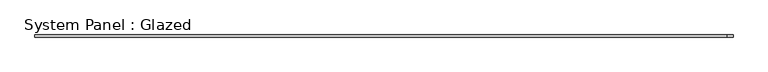
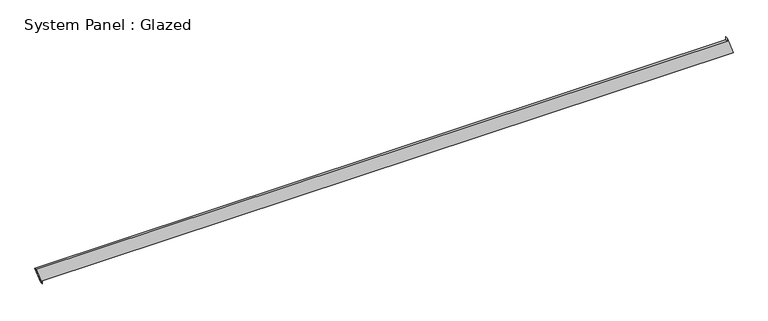
"""IFC4 building model written with IfcOpenShell, lengths in millimetres: plate geometry, System Panel : Glazed."""

import ifcopenshell
import ifcopenshell.guid

model = None  # the IFC model being written
_history = None  # IfcOwnerHistory: only IFC2X3 demands one
_inside = {}  # id of a spatial element -> (the spatial element, [elements in it])
_under = {}  # id of a project, library or spatial element -> (it, [spatial elements below it])
_declared = {}  # id of a project -> (the project, [libraries it declares])
_typed = {}  # id of a type object -> (the type object, [elements of that type])
_made_of = {}  # id of a material, layer set ... -> (it, [elements and type objects made of it])


def new_model(schema):
    """Start an empty IFC model of exactly this schema.

    Asked for "IFC4X3", IfcOpenShell would pick the latest addendum, in which some entities
    have other attributes; the version numbers below select the first issue.
    IFC2X3 requires an IfcOwnerHistory on every rooted entity: one is made here for all.
    """
    global model, _history
    if schema == "IFC4X3":
        model = ifcopenshell.file(schema_version=(4, 3, 0, 0))
    else:
        model = ifcopenshell.file(schema=schema)
    _inside.clear()
    _under.clear()
    _declared.clear()
    _typed.clear()
    _made_of.clear()
    _history = None
    if model.schema == "IFC2X3":
        org = make("IfcOrganization", Name="unknown")
        user = make(
            "IfcPersonAndOrganization",
            ThePerson=make("IfcPerson", FamilyName="unknown"),
            TheOrganization=org,
        )
        app = make(
            "IfcApplication",
            ApplicationDeveloper=org,
            Version="unknown",
            ApplicationFullName="unknown",
            ApplicationIdentifier="unknown",
        )
        _history = make(
            "IfcOwnerHistory",
            OwningUser=user,
            OwningApplication=app,
            ChangeAction="ADDED",
            CreationDate=0,
        )
    return model


def make(cls, **values):
    """One entity of the class cls with the attributes given. An attribute that is None is left unset."""
    return model.create_entity(
        cls, **{name: value for name, value in values.items() if value is not None}
    )


def rooted(cls, **values):
    """An entity with a GlobalId (a new one), such as an element, a storey or a relation."""
    return make(cls, GlobalId=ifcopenshell.guid.new(), OwnerHistory=_history, **values)


def si_unit(unit_type, name, prefix=None):
    """IfcSIUnit, for example si_unit("LENGTHUNIT", "METRE", prefix="MILLI")."""
    return make("IfcSIUnit", UnitType=unit_type, Prefix=prefix, Name=name)


def assignment(units):
    """IfcUnitAssignment: the units of a project."""
    return None if units is None else make("IfcUnitAssignment", Units=units)


def point(xyz):
    """IfcCartesianPoint."""
    return None if xyz is None else make("IfcCartesianPoint", Coordinates=xyz)


def direction(xyz):
    """IfcDirection."""
    return None if xyz is None else make("IfcDirection", DirectionRatios=xyz)


def frame(location, z_axis=None, x_axis=None):
    """IfcAxis2Placement3D, a coordinate frame: its origin and axes. An axis left out is left unset."""
    return make(
        "IfcAxis2Placement3D",
        Location=point(location),
        Axis=direction(z_axis),
        RefDirection=direction(x_axis),
    )


def origin():
    """The frame at (0, 0, 0) with its axes left unset."""
    return frame((0.0, 0.0, 0.0))


def place(relative_to, where):
    """IfcLocalPlacement: puts the frame where relative to a parent placement (None: the world)."""
    return make(
        "IfcLocalPlacement", PlacementRelTo=relative_to, RelativePlacement=where
    )


def context(
    kind, dimensions, precision=None, world=None, true_north=None, identifier=None
):
    """IfcGeometricRepresentationContext, for example the 3D "Model" context."""
    return make(
        "IfcGeometricRepresentationContext",
        ContextIdentifier=identifier,
        ContextType=kind,
        CoordinateSpaceDimension=dimensions,
        Precision=precision,
        WorldCoordinateSystem=world,
        TrueNorth=true_north,
    )


def project(units=None, contexts=None):
    """IfcProject with its units and contexts."""
    return rooted(
        "IfcProject",
        Name="project",
        RepresentationContexts=contexts,
        UnitsInContext=assignment(units),
    )


def spatial(cls, under=None, at=None, **own):
    """A site, building, storey or space (cls), placed at a placement, below another one or the project."""
    s = rooted(cls, ObjectPlacement=at, **own)
    if under is not None:
        _under.setdefault(under.id(), (under, []))[1].append(s)
    return s


def polyline(points):
    """IfcPolyline through the points."""
    return make("IfcPolyline", Points=[point(p) for p in points])


def outline(outer, holes=None, kind="AREA"):
    """IfcArbitraryClosedProfileDef: a profile drawn as a closed curve; with holes, ...WithVoids."""
    if holes is None:
        return make("IfcArbitraryClosedProfileDef", ProfileType=kind, OuterCurve=outer)
    return make(
        "IfcArbitraryProfileDefWithVoids",
        ProfileType=kind,
        OuterCurve=outer,
        InnerCurves=holes,
    )


def extrude(swept, where, along, depth):
    """IfcExtrudedAreaSolid: the profile swept, set in the frame where, extruded along a direction by depth."""
    return make(
        "IfcExtrudedAreaSolid",
        SweptArea=swept,
        Position=where,
        ExtrudedDirection=direction(along),
        Depth=depth,
    )


def shape(context_of_items, identifier, shape_type, items):
    """IfcShapeRepresentation: the items that make up one representation, for example the "Body"."""
    return make(
        "IfcShapeRepresentation",
        ContextOfItems=context_of_items,
        RepresentationIdentifier=identifier,
        RepresentationType=shape_type,
        Items=items,
    )


def source(mapping_origin, context_of_items, identifier, shape_type, items):
    """IfcRepresentationMap: a shape defined once, which mapped items show again and again."""
    return make(
        "IfcRepresentationMap",
        MappingOrigin=mapping_origin,
        MappedRepresentation=shape(context_of_items, identifier, shape_type, items),
    )


def transform(
    local_origin,
    x_axis=None,
    y_axis=None,
    z_axis=None,
    scale=None,
    scale2=None,
    scale3=None,
    uniform=True,
):
    """IfcCartesianTransformationOperator3D, or its non-uniform kind. x_axis, y_axis, z_axis: its Axis1, 2, 3."""
    if uniform:
        return make(
            "IfcCartesianTransformationOperator3D",
            Axis1=direction(x_axis),
            Axis2=direction(y_axis),
            LocalOrigin=point(local_origin),
            Scale=scale,
            Axis3=direction(z_axis),
        )
    return make(
        "IfcCartesianTransformationOperator3DnonUniform",
        Axis1=direction(x_axis),
        Axis2=direction(y_axis),
        LocalOrigin=point(local_origin),
        Scale=scale,
        Axis3=direction(z_axis),
        Scale2=scale2,
        Scale3=scale3,
    )


def mapped(mapping_source, mapping_target):
    """IfcMappedItem: shows the shape of a source again, moved by a transform."""
    return make(
        "IfcMappedItem", MappingSource=mapping_source, MappingTarget=mapping_target
    )


def made_of(thing, what):
    """Note that an element or type object is made of a material, layer set ...; save() writes the relation."""
    if what is not None:
        _made_of.setdefault(what.id(), (what, []))[1].append(thing)
    return thing


def element(
    cls,
    number,
    at=None,
    inside=None,
    cuts=None,
    type_object=None,
    material=None,
    context=None,
    identifier="Body",
    shape_type=None,
    held_by="IfcProductDefinitionShape",
    body=None,
    shapes=None,
    **own,
):
    """One element of the class cls, such as IfcWall. Its Tag is "e" and its number.

    at: its placement. inside: the storey or other place that contains it. cuts: it is an
    opening in that element (IfcRelVoidsElement). A single representation is given by context,
    identifier, shape_type and body (its items); several are given by shapes. held_by: the class
    of the entity that holds the representations. save() writes the other relations.
    """
    e = rooted(cls, Tag="e%d" % number, ObjectPlacement=at, **own)
    if body is not None:
        shapes = [shape(context, identifier, shape_type, body)]
    if shapes is not None:
        e.Representation = make(held_by, Representations=shapes)
    if inside is not None:
        _inside.setdefault(inside.id(), (inside, []))[1].append(e)
    if cuts is not None:
        rooted(
            "IfcRelVoidsElement", RelatingBuildingElement=cuts, RelatedOpeningElement=e
        )
    if type_object is not None:
        _typed.setdefault(type_object.id(), (type_object, []))[1].append(e)
    return made_of(e, material)


def aggregate(whole, parts):
    """IfcRelAggregates: a whole, such as a stair, and the parts it consists of."""
    return rooted("IfcRelAggregates", RelatingObject=whole, RelatedObjects=parts)


def save(model, path):
    """Write the relations noted so far, then the file.

    IfcRelAggregates (storeys below a building ...), IfcRelContainedInSpatialStructure (elements
    in a storey), IfcRelDefinesByType, IfcRelAssociatesMaterial and IfcRelDeclares: one each for
    every whole, place, type object, material and project.
    """
    for whole, parts in _under.values():
        aggregate(whole, parts)
    for where, things in _inside.values():
        rooted(
            "IfcRelContainedInSpatialStructure",
            RelatedElements=things,
            RelatingStructure=where,
        )
    for kind, things in _typed.values():
        rooted("IfcRelDefinesByType", RelatedObjects=things, RelatingType=kind)
    for what, things in _made_of.values():
        rooted("IfcRelAssociatesMaterial", RelatedObjects=things, RelatingMaterial=what)
    for by, libraries in _declared.values():
        rooted("IfcRelDeclares", RelatingContext=by, RelatedDefinitions=libraries)
    model.write(path)


def system_panel_glazed_3920cfb5(model_context):
    return source(origin(), model_context, "Body", "SweptSolid", [
        extrude(outline(polyline([(0.0, -3957.1612499), (35.3553391, -3957.1612499), (35.3553391, 4027.0933919), (235.3468796, 3957.4323455), (199.9915406, 3957.4328486), (199.8779154, -4027.0933919), (0.0, -3957.1612499)])), frame((0.0, -49.5, 0.0), z_axis=(0.0, 1.0, 0.0), x_axis=(0.0, 0.0, 1.0)), (0.0, 0.0, 1.0), 25.0),
    ])


if __name__ == "__main__":
    model = new_model("IFC4")
    model_context = context("Model", 3, world=origin())
    ifc_project = project(units=[si_unit("LENGTHUNIT", "METRE", prefix="MILLI")], contexts=[model_context])
    site = spatial("IfcSite", under=ifc_project)
    building = spatial("IfcBuilding", under=site)
    placement = place(None, origin())
    system_panel_glazed_shape = system_panel_glazed_3920cfb5(model_context)
    element("IfcPlate", 1, ObjectType="System Panel : Glazed", at=placement, inside=building, context=model_context, shape_type="MappedRepresentation", body=[
        mapped(system_panel_glazed_shape, transform((0.0, 0.0, 0.0), x_axis=(1.0, 0.0, 0.0), y_axis=(0.0, 1.0, 0.0), z_axis=(0.0, 0.0, 1.0))),
    ])
    save(model, "model.ifc")

# Revit data of these elements
# Element 1 (IfcPlate, "System Panel : Glazed")
#   Materials on its faces: "Glass"
# Materials
#   "Glass": class "Glass", colour RGB 218 227 224, transparency 0.85, Description = "Soda Lime Glass", Cost = 0
